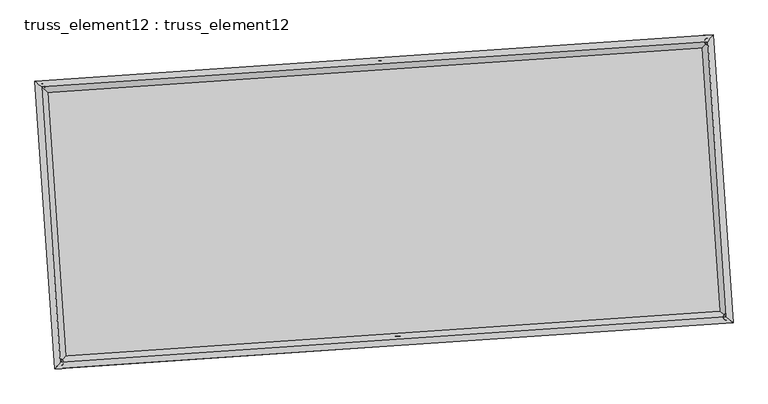
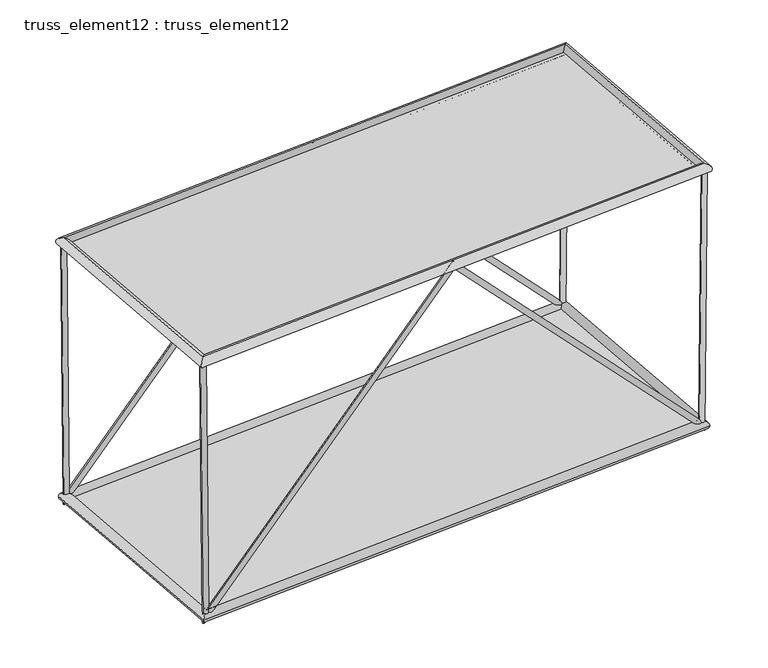
"""IFC4 building model written with IfcOpenShell, lengths in millimetres: plate geometry, truss_element12 : truss_element12."""

from ifc_helpers import new_model, si_unit, frame, origin, origin_with_axes, place, context, project, spatial, polyline, circle_curve, ellipse_curve, outline, extrude, source, transform, mapped, element, save
from ifc_brep_helpers import plane_surface, cylinder_surface, advanced_brep


def truss_element12_truss_element12_e15fa0d1(model_context):
    return source(origin(), model_context, "Body", "SolidModel", [
        advanced_brep(
        [(-3713.4759961, 2272.9146129, 5000.2487537), (-3812.5746463, 2259.5536584, 4999.2779762), (-3666.1330042, 2276.1427516, 122.9648409), (-3762.8538787, 2262.9439285, -122.9648409), (1063.2987247, 2598.6247229, 5071.8896074), (1063.7532103, 2592.0519183, 4927.6451965), (5793.5514433, 2921.1626744, 122.9707312), (5891.2095337, 2921.2178141, -122.9707312), (5840.0796469, 2924.3352558, 5000.2484753), (5940.0748654, 2924.5497553, 4999.2944025)],
        [
            (0, 1, circle_curve(frame((-3763.0253212, 2266.2341357, 4999.763365), z_axis=(-0.009706375954596178, -0.0006618408789575117, 0.999952672996317), x_axis=(-0.13360964715652263, 0.9910338295536035, -0.0006409891017273432)), 50.0)),
            (1, 0, circle_curve(frame((-3763.0253212, 2266.2341357, 4999.763365), z_axis=(-0.009706375954596178, -0.0006618408789575117, 0.999952672996317), x_axis=(-0.13360964715652263, 0.9910338295536035, -0.0006409891017273432)), 50.0)),
            (0, 2),
            (2, 3, ellipse_curve(frame((-3714.4934414, 2269.54334, 0.0), z_axis=(-0.9275912472386761, -0.0632489210447657, 0.36820381860169576), x_axis=(0.3673508361902778, 0.02504825708855167, 0.9297450983829544)), 132.5444982, 50.0)),
            (3, 1),
            (3, 2, ellipse_curve(frame((-3714.4934414, 2269.54334, 0.0), z_axis=(-0.9275912472386761, -0.0632489210447657, 0.36820381860169576), x_axis=(0.3673508361902778, 0.02504825708855167, 0.9297450983829544)), 132.5444982, 50.0)),
            (2, 4),
            (4, 5, ellipse_curve(frame((1063.5259675, 2595.3383206, 4999.7674019), z_axis=(-0.9976833951243606, -0.06802823816389074, -4.365141464700811e-05), x_axis=(4.355029160837673e-05, 2.9695288372236332e-06, -0.999999999047277)), 72.279252, 50.0)),
            (5, 3),
            (5, 4, ellipse_curve(frame((1063.5259675, 2595.3383206, 4999.7674019), z_axis=(-0.9976833951243606, -0.06802823816389074, -4.365141464700811e-05), x_axis=(4.355029160837673e-05, 2.9695288372236332e-06, -0.999999999047277)), 72.279252, 50.0)),
            (4, 6),
            (6, 7, ellipse_curve(frame((5842.3804885, 2921.1902443, 0.0), z_axis=(-0.927544453754612, -0.06324573037496357, -0.36832222835228934), x_axis=(-0.3674689716323779, -0.02505631229527868, 0.9296981962452138)), 132.5575344, 50.0)),
            (7, 5),
            (7, 6, ellipse_curve(frame((5842.3804885, 2921.1902443, 0.0), z_axis=(-0.927544453754612, -0.06324573037496357, -0.36832222835228934), x_axis=(-0.3674689716323779, -0.02505631229527868, 0.9296981962452138)), 132.5575344, 50.0)),
            (8, 9, circle_curve(frame((5890.0772562, 2924.4425055, 4999.7714389), z_axis=(0.009539353531430879, 0.0006504522548279124, 0.9999542877782297), x_axis=(-0.0021511031285793634, 0.9999974879501599, -0.000629959284471862)), 50.0)),
            (9, 8, circle_curve(frame((5890.0772562, 2924.4425055, 4999.7714389), z_axis=(0.009539353531430879, 0.0006504522548279124, 0.9999542877782297), x_axis=(-0.0021511031285793634, 0.9999974879501599, -0.000629959284471862)), 50.0)),
            (6, 8),
            (9, 7),
        ],
        [
            plane_surface(frame((-3763.0253212, 2316.2341247, 4999.7964586), z_axis=(-0.009706375954597944, -0.0006618408789585391, 0.999952672996317), x_axis=(0.9999528920233334, -6.424379033198588e-06, 0.009706373828539224))),
            cylinder_surface(frame((-3763.0253212, 2266.2341357, 4999.763365), z_axis=(-0.009706375954596176, -0.0006618408789575116, 0.9999526729963167), x_axis=(-0.13360964715652263, 0.9910338295536035, -0.0006409891017273432)), 50.0),
            cylinder_surface(frame((-3714.4934414, 2269.54334, 0.0), z_axis=(-0.6901274608072392, -0.04705716813236338, -0.7221562924790693), x_axis=(-0.020411412589058583, 0.9987523868619846, -0.045574597898475885)), 50.0),
            cylinder_surface(frame((1063.5259675, 2595.3383206, 4999.7674019), z_axis=(-0.6901903584114266, -0.04706145688090051, 0.7220958997475017), x_axis=(-0.11534547408446819, 0.9922791940867655, -0.045578751526874135)), 50.0),
            plane_surface(frame((5890.0772562, 2874.4425161, 4999.803963), z_axis=(0.009539353531431769, 0.000650452254824749, 0.9999542877782298), x_axis=(0.9999544993319458, -6.20517635319118e-06, -0.00953935151325425))),
            cylinder_surface(frame((5842.3804885, 2921.1902443, 0.0), z_axis=(-0.009539353531430879, -0.0006504522548279124, -0.9999542877782297), x_axis=(-0.0021511031285793634, 0.9999974879501599, -0.000629959284471862)), 50.0),
        ],
        [
            (0, [[1, 2]]),
            (1, [[-1, 3, 4, 5]]),
            (1, [[-2, -5, 6, -3]]),
            (2, [[-4, 7, 8, 9]]),
            (2, [[-6, -9, 10, -7]]),
            (3, [[-8, 11, 12, 13]]),
            (3, [[-10, -13, 14, -11]]),
            (4, [[15, 16]]),
            (5, [[-12, 17, -16, 18]]),
            (5, [[-14, -18, -15, -17]]),
        ],
    ),
        advanced_brep(
        [(-3441.3630431, -1717.8189714, 5000.2487537), (-3540.4616934, -1731.1799259, 4999.2779762), (-3394.0200512, -1714.5908327, 122.9648409), (-3490.7409258, -1727.7896558, -122.9648409), (1335.4116776, -1392.1088614, 5071.8896074), (1335.8661632, -1398.681666, 4927.6451965), (6065.6643962, -1069.5709099, 122.9707312), (6163.3224866, -1069.5157702, -122.9707312), (6112.1925998, -1066.3983285, 5000.2484753), (6212.1878184, -1066.183829, 4999.2944025)],
        [
            (0, 1, circle_curve(frame((-3490.9123683, -1724.4994486, 4999.763365), z_axis=(-0.009706375954596135, -0.0006618408789575164, 0.9999526729963168), x_axis=(-0.13360964715652227, 0.9910338295536036, -0.0006409891017273294)), 50.0)),
            (1, 0, circle_curve(frame((-3490.9123683, -1724.4994486, 4999.763365), z_axis=(-0.009706375954596135, -0.0006618408789575164, 0.9999526729963168), x_axis=(-0.13360964715652227, 0.9910338295536036, -0.0006409891017273294)), 50.0)),
            (0, 2),
            (2, 3, ellipse_curve(frame((-3442.3804885, -1721.1902443, 0.0), z_axis=(-0.9275912472386759, -0.06324892104476554, 0.3682038186016959), x_axis=(0.367350836190278, 0.025048257088551608, 0.9297450983829544)), 132.5444982, 50.0)),
            (3, 1),
            (3, 2, ellipse_curve(frame((-3442.3804885, -1721.1902443, 0.0), z_axis=(-0.9275912472386759, -0.06324892104476554, 0.3682038186016959), x_axis=(0.367350836190278, 0.025048257088551608, 0.9297450983829544)), 132.5444982, 50.0)),
            (2, 4),
            (4, 5, ellipse_curve(frame((1335.6389204, -1395.3952637, 4999.7674019), z_axis=(-0.9976833951243606, -0.06802823816389082, -4.365141464756978e-05), x_axis=(4.3550291608837996e-05, 2.9695288375022965e-06, -0.999999999047277)), 72.279252, 50.0)),
            (5, 3),
            (5, 4, ellipse_curve(frame((1335.6389204, -1395.3952637, 4999.7674019), z_axis=(-0.9976833951243606, -0.06802823816389082, -4.365141464756978e-05), x_axis=(4.3550291608837996e-05, 2.9695288375022965e-06, -0.999999999047277)), 72.279252, 50.0)),
            (4, 6),
            (6, 7, ellipse_curve(frame((6114.4934414, -1069.54334, 0.0), z_axis=(-0.9275444537546116, -0.06324573037496363, -0.3683222283522902), x_axis=(-0.36746897163237896, -0.025056312295278976, 0.9296981962452135)), 132.5575344, 50.0)),
            (7, 5),
            (7, 6, ellipse_curve(frame((6114.4934414, -1069.54334, 0.0), z_axis=(-0.9275444537546116, -0.06324573037496363, -0.3683222283522902), x_axis=(-0.36746897163237896, -0.025056312295278976, 0.9296981962452135)), 132.5575344, 50.0)),
            (8, 9, circle_curve(frame((6162.1902091, -1066.2910788, 4999.7714389), z_axis=(0.00953935353143073, 0.0006504522548277286, 0.9999542877782298), x_axis=(-0.002151103128579773, 0.99999748795016, -0.0006299592844716747)), 50.0)),
            (9, 8, circle_curve(frame((6162.1902091, -1066.2910788, 4999.7714389), z_axis=(0.00953935353143073, 0.0006504522548277286, 0.9999542877782298), x_axis=(-0.002151103128579773, 0.99999748795016, -0.0006299592844716747)), 50.0)),
            (6, 8),
            (9, 7),
        ],
        [
            plane_surface(frame((-3490.9123683, -1674.4994596, 4999.7964586), z_axis=(-0.009706375954594393, -0.0006618408789585428, 0.9999526729963171), x_axis=(0.9999528920233334, -6.424379033198588e-06, 0.009706373828535671))),
            cylinder_surface(frame((-3490.9123683, -1724.4994486, 4999.763365), z_axis=(-0.009706375954596135, -0.0006618408789575164, 0.9999526729963168), x_axis=(-0.13360964715652227, 0.9910338295536036, -0.0006409891017273294)), 50.0),
            cylinder_surface(frame((-3442.3804885, -1721.1902443, 0.0), z_axis=(-0.6901274608072394, -0.04705716813236327, -0.7221562924790689), x_axis=(-0.02041141258905865, 0.9987523868619846, -0.045574597898475684)), 50.0),
            cylinder_surface(frame((1335.6389204, -1395.3952637, 4999.7674019), z_axis=(-0.6901903584114277, -0.04706145688090081, 0.7220958997475004), x_axis=(-0.1153454740844682, 0.9922791940867656, -0.045578751526874)), 50.0),
            plane_surface(frame((6162.1902091, -1116.2910682, 4999.803963), z_axis=(0.009539353531431769, 0.0006504522548247543, 0.9999542877782298), x_axis=(0.9999544993319458, -6.205176353635269e-06, -0.00953935151325425))),
            cylinder_surface(frame((6114.4934414, -1069.54334, 0.0), z_axis=(-0.00953935353143073, -0.0006504522548277286, -0.9999542877782298), x_axis=(-0.002151103128579773, 0.99999748795016, -0.0006299592844716747)), 50.0),
        ],
        [
            (0, [[1, 2]]),
            (1, [[-1, 3, 4, 5]]),
            (1, [[-2, -5, 6, -3]]),
            (2, [[-4, 7, 8, 9]]),
            (2, [[-6, -9, 10, -7]]),
            (3, [[-8, 11, 12, 13]]),
            (3, [[-10, -13, 14, -11]]),
            (4, [[15, 16]]),
            (5, [[-12, 17, -16, 18]]),
            (5, [[-14, -18, -15, -17]]),
        ],
    ),
        advanced_brep(
        [(-3490.9102431, -1724.4970932, 4909.763365), (-3490.9144935, -1724.5018041, 5089.763365), (-3763.0277465, 2266.2361808, 5089.763365), (-3763.0228959, 2266.2320905, 4909.763365), (5890.0792315, 2924.4448507, 5089.7714389), (5890.0752808, 2924.4401603, 4909.7714389), (6162.1924845, -1066.2931342, 5089.7714389), (6162.1879337, -1066.2890234, 4909.7714389)],
        [
            (0, 1, ellipse_curve(frame((-3490.9123683, -1724.4994486, 4999.763365), z_axis=(-0.7535719234052112, 0.6573654662780987, -5.900580049914557e-07), x_axis=(-0.6573654662778362, -0.7535719234054403, -5.900580049915072e-07)), 127.2792206, 90.0)),
            (1, 2),
            (2, 3, ellipse_curve(frame((-3763.0253212, 2266.2341357, 4999.763365), z_axis=(-0.6573654662778363, -0.7535719234054402, -5.900580037253456e-07), x_axis=(0.7535719234052112, -0.6573654662780987, 5.90058003725294e-07)), 127.2792206, 90.0)),
            (3, 0),
            (1, 0, ellipse_curve(frame((-3490.9123683, -1724.4994486, 4999.763365), z_axis=(-0.7535719234052112, 0.6573654662780987, -5.900580049914557e-07), x_axis=(-0.6573654662778362, -0.7535719234054403, -5.900580049915072e-07)), 127.2792206, 90.0)),
            (3, 2, ellipse_curve(frame((-3763.0253212, 2266.2341357, 4999.763365), z_axis=(-0.6573654662778363, -0.7535719234054402, -5.900580037253456e-07), x_axis=(0.7535719234052112, -0.6573654662780987, 5.90058003725294e-07)), 127.2792206, 90.0)),
            (2, 4),
            (4, 5, ellipse_curve(frame((5890.0772562, 2924.4425055, 4999.7714389), z_axis=(-0.7535719234052125, 0.6573654662780972, -5.900580067881512e-07), x_axis=(-0.657365466277835, -0.7535719234054412, -5.900580006624883e-07)), 127.2792206, 90.0)),
            (5, 3),
            (5, 4, ellipse_curve(frame((5890.0772562, 2924.4425055, 4999.7714389), z_axis=(-0.7535719234052125, 0.6573654662780972, -5.900580067881512e-07), x_axis=(-0.657365466277835, -0.7535719234054412, -5.900580006624883e-07)), 127.2792206, 90.0)),
            (4, 6),
            (6, 7, ellipse_curve(frame((6162.1902091, -1066.2910788, 4999.7714389), z_axis=(0.6573654662778348, 0.7535719234054415, 5.9005800192865e-07), x_axis=(-0.7535719234052125, 0.6573654662780972, -5.90058008054313e-07)), 127.2792206, 90.0)),
            (7, 5),
            (7, 6, ellipse_curve(frame((6162.1902091, -1066.2910788, 4999.7714389), z_axis=(0.6573654662778348, 0.7535719234054415, 5.9005800192865e-07), x_axis=(-0.7535719234052125, 0.6573654662780972, -5.90058008054313e-07)), 127.2792206, 90.0)),
            (6, 1),
            (0, 7),
        ],
        [
            cylinder_surface(frame((-3490.9123683, -1724.4994486, 4999.763365), z_axis=(0.06802823822869981, -0.9976833960748768, 0.0), x_axis=(-0.997683395754587, -0.06802823820686048, -2.5339041105448512e-05)), 90.0),
            cylinder_surface(frame((-3763.0253212, 2266.2341357, 4999.763365), z_axis=(-0.9976833960745294, -0.06802823822867587, -8.344680314551415e-07), x_axis=(-0.06802823818787405, 0.9976833957767263, -2.4504573074243944e-05)), 90.0),
            cylinder_surface(frame((5890.0772562, 2924.4425055, 4999.7714389), z_axis=(-0.0680282382287038, 0.9976833960748765, 0.0), x_axis=(0.9976833957953886, 0.06802823820964657, -2.3670105038707918e-05)), 90.0),
            cylinder_surface(frame((6162.1902091, -1066.2910788, 4999.7714389), z_axis=(0.9976833960745295, 0.0680282382286759, 8.344680332457648e-07), x_axis=(0.0680282382286759, -0.9976833957739443, -2.4504573067371715e-05)), 90.0),
        ],
        [
            (0, [[1, 2, 3, 4]]),
            (0, [[5, -4, 6, -2]]),
            (1, [[-3, 7, 8, 9]]),
            (1, [[-6, -9, 10, -7]]),
            (2, [[-8, 11, 12, 13]]),
            (2, [[-10, -13, 14, -11]]),
            (3, [[-12, 15, -1, 16]]),
            (3, [[-14, -16, -5, -15]]),
        ],
    ),
        advanced_brep(
        [(-3358.7115243, -1625.2761972, 0.0), (-3526.0494527, -1817.1042913, 0.0), (-3810.4074885, 2353.2123043, 0.0), (-3618.5793943, 2185.8743758, 0.0), (5926.0494527, 3017.1042913, 0.0), (5758.7115243, 2825.2761972, 0.0), (6210.4074885, -1153.2123043, 0.0), (6018.5793943, -985.8743758, 0.0)],
        [
            (0, 1, ellipse_curve(frame((-3442.3804885, -1721.1902443, 0.0), z_axis=(-0.7535719234054589, 0.6573654662780798, 0.0), x_axis=(-0.6573654662780798, -0.753571923405459, 0.0)), 127.2792206, 90.0)),
            (1, 2),
            (2, 3, ellipse_curve(frame((-3714.4934414, 2269.54334, 0.0), z_axis=(-0.6573654662780798, -0.7535719234054588, 0.0), x_axis=(0.7535719234054586, -0.6573654662780799, 0.0)), 127.2792206, 90.0)),
            (3, 0),
            (1, 0, ellipse_curve(frame((-3442.3804885, -1721.1902443, 0.0), z_axis=(-0.7535719234054589, 0.6573654662780798, 0.0), x_axis=(-0.6573654662780798, -0.753571923405459, 0.0)), 127.2792206, 90.0)),
            (3, 2, ellipse_curve(frame((-3714.4934414, 2269.54334, 0.0), z_axis=(-0.6573654662780798, -0.7535719234054588, 0.0), x_axis=(0.7535719234054586, -0.6573654662780799, 0.0)), 127.2792206, 90.0)),
            (2, 4),
            (4, 5, ellipse_curve(frame((5842.3804885, 2921.1902443, 0.0), z_axis=(-0.7535719234054601, 0.6573654662780783, 0.0), x_axis=(-0.6573654662780783, -0.7535719234054601, 0.0)), 127.2792206, 90.0)),
            (5, 3),
            (5, 4, ellipse_curve(frame((5842.3804885, 2921.1902443, 0.0), z_axis=(-0.7535719234054601, 0.6573654662780783, 0.0), x_axis=(-0.6573654662780783, -0.7535719234054601, 0.0)), 127.2792206, 90.0)),
            (4, 6),
            (6, 7, ellipse_curve(frame((6114.4934414, -1069.54334, 0.0), z_axis=(0.6573654662780781, 0.7535719234054602, 0.0), x_axis=(-0.75357192340546, 0.6573654662780785, 0.0)), 127.2792206, 90.0)),
            (7, 5),
            (7, 6, ellipse_curve(frame((6114.4934414, -1069.54334, 0.0), z_axis=(0.6573654662780781, 0.7535719234054602, 0.0), x_axis=(-0.75357192340546, 0.6573654662780785, 0.0)), 127.2792206, 90.0)),
            (6, 1),
            (0, 7),
        ],
        [
            cylinder_surface(frame((-3442.3804885, -1721.1902443, 0.0), z_axis=(0.06802823822870269, -0.9976833960748767, 0.0), x_axis=(-0.9976833960748767, -0.06802823822870269, 0.0)), 90.0),
            cylinder_surface(frame((-3714.4934414, 2269.54334, 0.0), z_axis=(-0.9976833960748765, -0.06802823822870226, 0.0), x_axis=(-0.06802823822870226, 0.9976833960748765, 0.0)), 90.0),
            cylinder_surface(frame((5842.3804885, 2921.1902443, 0.0), z_axis=(-0.06802823822870668, 0.9976833960748762, 0.0), x_axis=(0.9976833960748762, 0.06802823822870668, 0.0)), 90.0),
            cylinder_surface(frame((6114.4934414, -1069.54334, 0.0), z_axis=(0.9976833960748765, 0.06802823822870253, 0.0), x_axis=(0.06802823822870253, -0.9976833960748765, 0.0)), 90.0),
        ],
        [
            (0, [[1, 2, 3, 4]]),
            (0, [[5, -4, 6, -2]]),
            (1, [[-3, 7, 8, 9]]),
            (1, [[-6, -9, 10, -7]]),
            (2, [[-8, 11, 12, 13]]),
            (2, [[-10, -13, 14, -11]]),
            (3, [[-12, 15, -1, 16]]),
            (3, [[-14, -16, -5, -15]]),
        ],
    ),
        extrude(outline(polyline([(-3442.3804885, -1721.1902443), (-3714.4934414, 2269.54334), (5842.3804885, 2921.1902443), (6114.4934414, -1069.54334), (-3442.3804885, -1721.1902443)])), origin_with_axes(), (0.0, 0.0, 1.0), 20.0),
        extrude(outline(polyline([(-1999.9999999, 4837.7584589), (2000.0000001, 4837.7584589), (2000.0, -4837.758459), (-2000.0, -4837.758459), (-1999.9999999, 4837.7584589)])), frame((1199.5824439, 599.9715284, 4999.7674019), z_axis=(-8.325348995380487e-07, -5.6767390038064906e-08, 0.9999999999996518), x_axis=(-0.06802823822870302, 0.9976833960748764, 0.0)), (0.0, 0.0, 1.0), 20.0),
    ])


if __name__ == "__main__":
    model = new_model("IFC4")
    model_context = context("Model", 3, world=origin())
    ifc_project = project(units=[si_unit("LENGTHUNIT", "METRE", prefix="MILLI")], contexts=[model_context])
    site = spatial("IfcSite", under=ifc_project)
    building = spatial("IfcBuilding", under=site)
    placement = place(None, origin())
    truss_element12_truss_element12_shape = truss_element12_truss_element12_e15fa0d1(model_context)
    element("IfcPlate", 1, ObjectType="truss_element12 : truss_element12", at=placement, inside=building, context=model_context, shape_type="MappedRepresentation", body=[
        mapped(truss_element12_truss_element12_shape, transform((0.0, 0.0, 0.0), x_axis=(1.0, 0.0, 0.0), y_axis=(0.0, 1.0, 0.0), z_axis=(0.0, 0.0, 1.0))),
    ])
    save(model, "model.ifc")

# Revit data of these elements
# Type "truss_element12 : truss_element12"
#   steellbar1 = 90 mm
#   steelbar2 = 50 mm
#   offset1 = 5000 mm
#   M = Default Roof
# Element 1 (IfcPlate, "truss_element12 : truss_element12")
#   Materials on its faces: "Default Roof"
# Materials
#   "Default Roof": class "Miscellaneous", colour RGB 0 127 0, transparency 0, Comments = "Rendering appearance not upgraded Rendering appearance not upgraded ", Cost = 0
